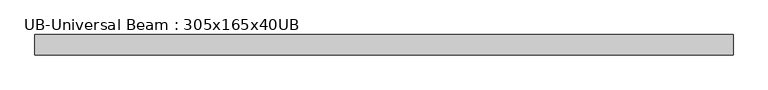
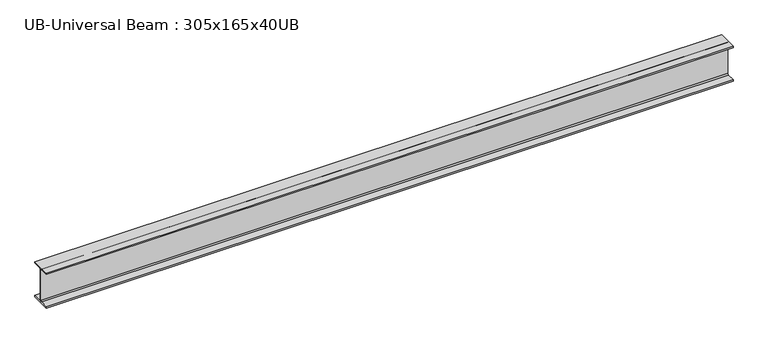
"""IFC4 building model written with IfcOpenShell, lengths in millimetres: beam geometry, UB-Universal Beam : 305x165x40UB."""

import ifcopenshell
import ifcopenshell.guid

model = None  # the IFC model being written
_history = None  # IfcOwnerHistory: only IFC2X3 demands one
_inside = {}  # id of a spatial element -> (the spatial element, [elements in it])
_under = {}  # id of a project, library or spatial element -> (it, [spatial elements below it])
_declared = {}  # id of a project -> (the project, [libraries it declares])
_typed = {}  # id of a type object -> (the type object, [elements of that type])
_made_of = {}  # id of a material, layer set ... -> (it, [elements and type objects made of it])


def new_model(schema):
    """Start an empty IFC model of exactly this schema.

    Asked for "IFC4X3", IfcOpenShell would pick the latest addendum, in which some entities
    have other attributes; the version numbers below select the first issue.
    IFC2X3 requires an IfcOwnerHistory on every rooted entity: one is made here for all.
    """
    global model, _history
    if schema == "IFC4X3":
        model = ifcopenshell.file(schema_version=(4, 3, 0, 0))
    else:
        model = ifcopenshell.file(schema=schema)
    _inside.clear()
    _under.clear()
    _declared.clear()
    _typed.clear()
    _made_of.clear()
    _history = None
    if model.schema == "IFC2X3":
        org = make("IfcOrganization", Name="unknown")
        user = make(
            "IfcPersonAndOrganization",
            ThePerson=make("IfcPerson", FamilyName="unknown"),
            TheOrganization=org,
        )
        app = make(
            "IfcApplication",
            ApplicationDeveloper=org,
            Version="unknown",
            ApplicationFullName="unknown",
            ApplicationIdentifier="unknown",
        )
        _history = make(
            "IfcOwnerHistory",
            OwningUser=user,
            OwningApplication=app,
            ChangeAction="ADDED",
            CreationDate=0,
        )
    return model


def make(cls, **values):
    """One entity of the class cls with the attributes given. An attribute that is None is left unset."""
    return model.create_entity(
        cls, **{name: value for name, value in values.items() if value is not None}
    )


def rooted(cls, **values):
    """An entity with a GlobalId (a new one), such as an element, a storey or a relation."""
    return make(cls, GlobalId=ifcopenshell.guid.new(), OwnerHistory=_history, **values)


def si_unit(unit_type, name, prefix=None):
    """IfcSIUnit, for example si_unit("LENGTHUNIT", "METRE", prefix="MILLI")."""
    return make("IfcSIUnit", UnitType=unit_type, Prefix=prefix, Name=name)


def assignment(units):
    """IfcUnitAssignment: the units of a project."""
    return None if units is None else make("IfcUnitAssignment", Units=units)


def point(xyz):
    """IfcCartesianPoint."""
    return None if xyz is None else make("IfcCartesianPoint", Coordinates=xyz)


def direction(xyz):
    """IfcDirection."""
    return None if xyz is None else make("IfcDirection", DirectionRatios=xyz)


def frame(location, z_axis=None, x_axis=None):
    """IfcAxis2Placement3D, a coordinate frame: its origin and axes. An axis left out is left unset."""
    return make(
        "IfcAxis2Placement3D",
        Location=point(location),
        Axis=direction(z_axis),
        RefDirection=direction(x_axis),
    )


def frame_2d(location, x_axis=None):
    """IfcAxis2Placement2D, a coordinate frame in the plane: its origin and x axis."""
    return make(
        "IfcAxis2Placement2D", Location=point(location), RefDirection=direction(x_axis)
    )


def origin():
    """The frame at (0, 0, 0) with its axes left unset."""
    return frame((0.0, 0.0, 0.0))


def place(relative_to, where):
    """IfcLocalPlacement: puts the frame where relative to a parent placement (None: the world)."""
    return make(
        "IfcLocalPlacement", PlacementRelTo=relative_to, RelativePlacement=where
    )


def context(
    kind, dimensions, precision=None, world=None, true_north=None, identifier=None
):
    """IfcGeometricRepresentationContext, for example the 3D "Model" context."""
    return make(
        "IfcGeometricRepresentationContext",
        ContextIdentifier=identifier,
        ContextType=kind,
        CoordinateSpaceDimension=dimensions,
        Precision=precision,
        WorldCoordinateSystem=world,
        TrueNorth=true_north,
    )


def project(units=None, contexts=None):
    """IfcProject with its units and contexts."""
    return rooted(
        "IfcProject",
        Name="project",
        RepresentationContexts=contexts,
        UnitsInContext=assignment(units),
    )


def spatial(cls, under=None, at=None, **own):
    """A site, building, storey or space (cls), placed at a placement, below another one or the project."""
    s = rooted(cls, ObjectPlacement=at, **own)
    if under is not None:
        _under.setdefault(under.id(), (under, []))[1].append(s)
    return s


def polyline(points):
    """IfcPolyline through the points."""
    return make("IfcPolyline", Points=[point(p) for p in points])


def circle_curve(where, radius):
    """IfcCircle in the frame where."""
    return make("IfcCircle", Position=where, Radius=radius)


def trimmed(basis, trim1, trim2, sense, master):
    """IfcTrimmedCurve: the piece of a basis curve between two trims."""
    return make(
        "IfcTrimmedCurve",
        BasisCurve=basis,
        Trim1=trim1,
        Trim2=trim2,
        SenseAgreement=sense,
        MasterRepresentation=master,
    )


def segment(curve, same_sense, transition):
    """IfcCompositeCurveSegment."""
    return make(
        "IfcCompositeCurveSegment",
        Transition=transition,
        SameSense=same_sense,
        ParentCurve=curve,
    )


def composite_curve(segments, self_intersect=None):
    """IfcCompositeCurve: segments joined end to end."""
    return make("IfcCompositeCurve", Segments=segments, SelfIntersect=self_intersect)


def outline(outer, holes=None, kind="AREA"):
    """IfcArbitraryClosedProfileDef: a profile drawn as a closed curve; with holes, ...WithVoids."""
    if holes is None:
        return make("IfcArbitraryClosedProfileDef", ProfileType=kind, OuterCurve=outer)
    return make(
        "IfcArbitraryProfileDefWithVoids",
        ProfileType=kind,
        OuterCurve=outer,
        InnerCurves=holes,
    )


def extrude(swept, where, along, depth):
    """IfcExtrudedAreaSolid: the profile swept, set in the frame where, extruded along a direction by depth."""
    return make(
        "IfcExtrudedAreaSolid",
        SweptArea=swept,
        Position=where,
        ExtrudedDirection=direction(along),
        Depth=depth,
    )


def shape(context_of_items, identifier, shape_type, items):
    """IfcShapeRepresentation: the items that make up one representation, for example the "Body"."""
    return make(
        "IfcShapeRepresentation",
        ContextOfItems=context_of_items,
        RepresentationIdentifier=identifier,
        RepresentationType=shape_type,
        Items=items,
    )


def source(mapping_origin, context_of_items, identifier, shape_type, items):
    """IfcRepresentationMap: a shape defined once, which mapped items show again and again."""
    return make(
        "IfcRepresentationMap",
        MappingOrigin=mapping_origin,
        MappedRepresentation=shape(context_of_items, identifier, shape_type, items),
    )


def transform(
    local_origin,
    x_axis=None,
    y_axis=None,
    z_axis=None,
    scale=None,
    scale2=None,
    scale3=None,
    uniform=True,
):
    """IfcCartesianTransformationOperator3D, or its non-uniform kind. x_axis, y_axis, z_axis: its Axis1, 2, 3."""
    if uniform:
        return make(
            "IfcCartesianTransformationOperator3D",
            Axis1=direction(x_axis),
            Axis2=direction(y_axis),
            LocalOrigin=point(local_origin),
            Scale=scale,
            Axis3=direction(z_axis),
        )
    return make(
        "IfcCartesianTransformationOperator3DnonUniform",
        Axis1=direction(x_axis),
        Axis2=direction(y_axis),
        LocalOrigin=point(local_origin),
        Scale=scale,
        Axis3=direction(z_axis),
        Scale2=scale2,
        Scale3=scale3,
    )


def mapped(mapping_source, mapping_target):
    """IfcMappedItem: shows the shape of a source again, moved by a transform."""
    return make(
        "IfcMappedItem", MappingSource=mapping_source, MappingTarget=mapping_target
    )


def made_of(thing, what):
    """Note that an element or type object is made of a material, layer set ...; save() writes the relation."""
    if what is not None:
        _made_of.setdefault(what.id(), (what, []))[1].append(thing)
    return thing


def element(
    cls,
    number,
    at=None,
    inside=None,
    cuts=None,
    type_object=None,
    material=None,
    context=None,
    identifier="Body",
    shape_type=None,
    held_by="IfcProductDefinitionShape",
    body=None,
    shapes=None,
    **own,
):
    """One element of the class cls, such as IfcWall. Its Tag is "e" and its number.

    at: its placement. inside: the storey or other place that contains it. cuts: it is an
    opening in that element (IfcRelVoidsElement). A single representation is given by context,
    identifier, shape_type and body (its items); several are given by shapes. held_by: the class
    of the entity that holds the representations. save() writes the other relations.
    """
    e = rooted(cls, Tag="e%d" % number, ObjectPlacement=at, **own)
    if body is not None:
        shapes = [shape(context, identifier, shape_type, body)]
    if shapes is not None:
        e.Representation = make(held_by, Representations=shapes)
    if inside is not None:
        _inside.setdefault(inside.id(), (inside, []))[1].append(e)
    if cuts is not None:
        rooted(
            "IfcRelVoidsElement", RelatingBuildingElement=cuts, RelatedOpeningElement=e
        )
    if type_object is not None:
        _typed.setdefault(type_object.id(), (type_object, []))[1].append(e)
    return made_of(e, material)


def aggregate(whole, parts):
    """IfcRelAggregates: a whole, such as a stair, and the parts it consists of."""
    return rooted("IfcRelAggregates", RelatingObject=whole, RelatedObjects=parts)


def save(model, path):
    """Write the relations noted so far, then the file.

    IfcRelAggregates (storeys below a building ...), IfcRelContainedInSpatialStructure (elements
    in a storey), IfcRelDefinesByType, IfcRelAssociatesMaterial and IfcRelDeclares: one each for
    every whole, place, type object, material and project.
    """
    for whole, parts in _under.values():
        aggregate(whole, parts)
    for where, things in _inside.values():
        rooted(
            "IfcRelContainedInSpatialStructure",
            RelatedElements=things,
            RelatingStructure=where,
        )
    for kind, things in _typed.values():
        rooted("IfcRelDefinesByType", RelatedObjects=things, RelatingType=kind)
    for what, things in _made_of.values():
        rooted("IfcRelAssociatesMaterial", RelatedObjects=things, RelatingMaterial=what)
    for by, libraries in _declared.values():
        rooted("IfcRelDeclares", RelatingContext=by, RelatedDefinitions=libraries)
    model.write(path)


def ub_universal_beam_305x165x40ub_26306981(model_context):
    return source(origin(), model_context, "Body", "SweptSolid", [
        extrude(outline(composite_curve([segment(polyline([(82.5, -141.5), (82.5, -151.7), (-82.5, -151.7), (-82.5, -141.5), (-11.9, -141.5)]), True, "CONTINUOUS"), segment(trimmed(circle_curve(frame_2d((-11.9, -132.6)), 8.9), [point((-11.9, -141.5))], [point((-3.0, -132.6))], True, "CARTESIAN"), True, "CONTINUOUS"), segment(polyline([(-3.0, -132.6), (-3.0, 132.6)]), True, "CONTINUOUS"), segment(trimmed(circle_curve(frame_2d((-11.9, 132.6)), 8.9), [point((-3.0, 132.6))], [point((-11.9, 141.5))], True, "CARTESIAN"), True, "CONTINUOUS"), segment(polyline([(-11.9, 141.5), (-82.5, 141.5), (-82.5, 151.7), (82.5, 151.7), (82.5, 141.5), (11.9, 141.5)]), True, "CONTINUOUS"), segment(trimmed(circle_curve(frame_2d((11.9, 132.6)), 8.9), [point((11.9, 141.5))], [point((3.0, 132.6))], True, "CARTESIAN"), True, "CONTINUOUS"), segment(polyline([(3.0, 132.6), (3.0, -132.6)]), True, "CONTINUOUS"), segment(trimmed(circle_curve(frame_2d((11.9, -132.6)), 8.9), [point((3.0, -132.6))], [point((11.9, -141.5))], True, "CARTESIAN"), True, "CONTINUOUS"), segment(polyline([(11.9, -141.5), (82.5, -141.5)]), True, "CONTINUOUS")], self_intersect=False)), frame((-2832.175, 0.0, 0.0), z_axis=(1.0, 0.0, 0.0), x_axis=(0.0, 1.0, 0.0)), (0.0, 0.0, 1.0), 5664.35),
    ])


if __name__ == "__main__":
    model = new_model("IFC4")
    model_context = context("Model", 3, world=origin())
    ifc_project = project(units=[si_unit("LENGTHUNIT", "METRE", prefix="MILLI")], contexts=[model_context])
    site = spatial("IfcSite", under=ifc_project)
    building = spatial("IfcBuilding", under=site)
    placement = place(None, origin())
    ub_universal_beam_305x165x40ub_shape = ub_universal_beam_305x165x40ub_26306981(model_context)
    element("IfcBeam", 1, ObjectType="UB-Universal Beam : 305x165x40UB", at=placement, inside=building, context=model_context, shape_type="MappedRepresentation", body=[
        mapped(ub_universal_beam_305x165x40ub_shape, transform((0.0, 0.0, 0.0), x_axis=(1.0, 0.0, 0.0), y_axis=(0.0, 1.0, 0.0), z_axis=(0.0, 0.0, 1.0))),
    ])
    save(model, "model.ifc")

# Revit data of these elements
# Project information
#   Project Issue Date = "October 2010"
#   Project Status = "Project Status"
#   Client Name = "Building CAD"
#   Project Address = "Enter address here"
#   Project Name = "Retail Units"
#   Project Number = "NA"
# Type "UB-Universal Beam : 305x165x40UB"
#   Nominal h = "305"
#   W = 0
#   Start Extension Calculation [instance default] = 3000 mm
#   Start Extension [instance default] = -12.7 mm
#   End Extension Calculation [instance default] = 3000 mm
#   End Extension [instance default] = -12.7 mm
#   Ix = 8503
#   Length [instance default] = 1524 mm
#   M = 40.3
#   Zx = 560
#   b = 165 mm
#   h = 303.4 mm
#   r = 8.9 mm
#   s = 6 mm
#   t = 10.2 mm
#   A = 0.005 m²
#   Structural Material [instance default] = Metal - Steel - 345 MPa
#   Assembly Code = ""
# Element 1 (IfcBeam, "UB-Universal Beam : 305x165x40UB")
#   Materials on its faces: "Metal - Steel - 345 MPa"
# Materials
#   "Metal - Steel - 345 MPa": class "Metal", colour RGB 241 46 46, transparency 0
